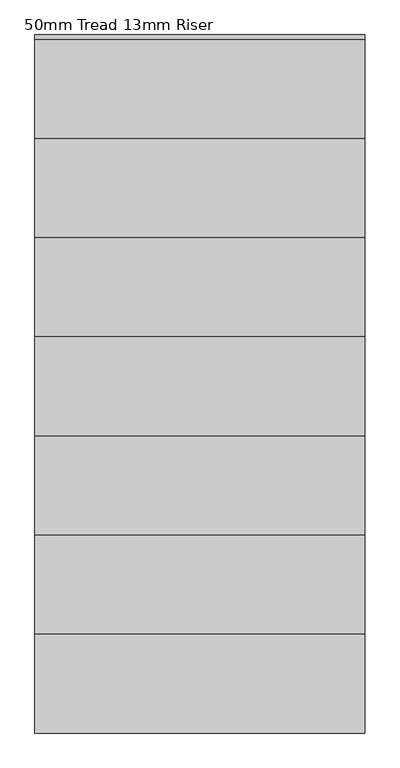
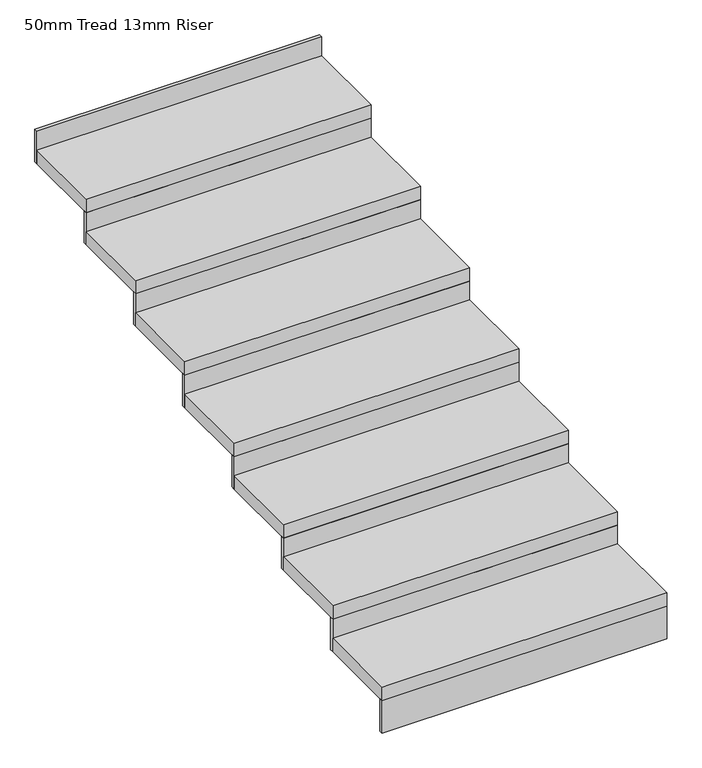
"""IFC4 building model written with IfcOpenShell, lengths in millimetres: stair flight geometry, 50mm Tread 13mm Riser."""

from ifc_helpers import new_model, si_unit, frame, origin, place, context, project, spatial, polyline, outline, extrude, source, transform, mapped, element, save


def stair_flight_50mm_tread_13mm_riser_fa5e52d7(model_context):
    return source(origin(), model_context, "Body", "SweptSolid", [
        extrude(outline(polyline([(22749.836337, -2886.2292651), (22749.836337, -2898.7292651), (21749.836337, -2898.7292651), (21749.836337, -2886.2292651), (22749.836337, -2886.2292651)])), frame((0.0, 0.0, 4630.0), z_axis=(0.0, 0.0, 1.0), x_axis=(1.0, 0.0, 0.0)), (0.0, 0.0, 1.0), 120.0),
        extrude(outline(polyline([(21749.836337, -2598.7292651), (22749.836337, -2598.7292651), (22749.836337, -2898.7292651), (21749.836337, -2898.7292651), (21749.836337, -2598.7292651)])), frame((0.0, 0.0, 4750.0), z_axis=(0.0, 0.0, 1.0), x_axis=(1.0, 0.0, 0.0)), (0.0, 0.0, 1.0), 50.0),
        extrude(outline(polyline([(22749.836337, -2586.2292651), (22749.836337, -2598.7292651), (21749.836337, -2598.7292651), (21749.836337, -2586.2292651), (22749.836337, -2586.2292651)])), frame((0.0, 0.0, 4750.0), z_axis=(0.0, 0.0, 1.0), x_axis=(1.0, 0.0, 0.0)), (0.0, 0.0, 1.0), 120.0),
        extrude(outline(polyline([(21749.836337, -2298.7292651), (22749.836337, -2298.7292651), (22749.836337, -2598.7292651), (21749.836337, -2598.7292651), (21749.836337, -2298.7292651)])), frame((0.0, 0.0, 4870.0), z_axis=(0.0, 0.0, 1.0), x_axis=(1.0, 0.0, 0.0)), (0.0, 0.0, 1.0), 50.0),
        extrude(outline(polyline([(22749.836337, -2286.2292651), (22749.836337, -2298.7292651), (21749.836337, -2298.7292651), (21749.836337, -2286.2292651), (22749.836337, -2286.2292651)])), frame((0.0, 0.0, 4870.0), z_axis=(0.0, 0.0, 1.0), x_axis=(1.0, 0.0, 0.0)), (0.0, 0.0, 1.0), 120.0),
        extrude(outline(polyline([(21749.836337, -1998.7292651), (22749.836337, -1998.7292651), (22749.836337, -2298.7292651), (21749.836337, -2298.7292651), (21749.836337, -1998.7292651)])), frame((0.0, 0.0, 4990.0), z_axis=(0.0, 0.0, 1.0), x_axis=(1.0, 0.0, 0.0)), (0.0, 0.0, 1.0), 50.0),
        extrude(outline(polyline([(22749.836337, -1986.2292651), (22749.836337, -1998.7292651), (21749.836337, -1998.7292651), (21749.836337, -1986.2292651), (22749.836337, -1986.2292651)])), frame((0.0, 0.0, 4990.0), z_axis=(0.0, 0.0, 1.0), x_axis=(1.0, 0.0, 0.0)), (0.0, 0.0, 1.0), 120.0),
        extrude(outline(polyline([(21749.836337, -1698.7292651), (22749.836337, -1698.7292651), (22749.836337, -1998.7292651), (21749.836337, -1998.7292651), (21749.836337, -1698.7292651)])), frame((0.0, 0.0, 5110.0), z_axis=(0.0, 0.0, 1.0), x_axis=(1.0, 0.0, 0.0)), (0.0, 0.0, 1.0), 50.0),
        extrude(outline(polyline([(22749.836337, -1686.2292651), (22749.836337, -1698.7292651), (21749.836337, -1698.7292651), (21749.836337, -1686.2292651), (22749.836337, -1686.2292651)])), frame((0.0, 0.0, 5110.0), z_axis=(0.0, 0.0, 1.0), x_axis=(1.0, 0.0, 0.0)), (0.0, 0.0, 1.0), 120.0),
        extrude(outline(polyline([(21749.836337, -1398.7292651), (22749.836337, -1398.7292651), (22749.836337, -1698.7292651), (21749.836337, -1698.7292651), (21749.836337, -1398.7292651)])), frame((0.0, 0.0, 5230.0), z_axis=(0.0, 0.0, 1.0), x_axis=(1.0, 0.0, 0.0)), (0.0, 0.0, 1.0), 50.0),
        extrude(outline(polyline([(22749.836337, -1386.2292651), (22749.836337, -1398.7292651), (21749.836337, -1398.7292651), (21749.836337, -1386.2292651), (22749.836337, -1386.2292651)])), frame((0.0, 0.0, 5230.0), z_axis=(0.0, 0.0, 1.0), x_axis=(1.0, 0.0, 0.0)), (0.0, 0.0, 1.0), 120.0),
        extrude(outline(polyline([(21749.836337, -1098.7292651), (22749.836337, -1098.7292651), (22749.836337, -1398.7292651), (21749.836337, -1398.7292651), (21749.836337, -1098.7292651)])), frame((0.0, 0.0, 5350.0), z_axis=(0.0, 0.0, 1.0), x_axis=(1.0, 0.0, 0.0)), (0.0, 0.0, 1.0), 50.0),
        extrude(outline(polyline([(22749.836337, -1086.2292651), (22749.836337, -1098.7292651), (21749.836337, -1098.7292651), (21749.836337, -1086.2292651), (22749.836337, -1086.2292651)])), frame((0.0, 0.0, 5350.0), z_axis=(0.0, 0.0, 1.0), x_axis=(1.0, 0.0, 0.0)), (0.0, 0.0, 1.0), 120.0),
        extrude(outline(polyline([(21749.836337, -798.7292651), (22749.836337, -798.7292651), (22749.836337, -1098.7292651), (21749.836337, -1098.7292651), (21749.836337, -798.7292651)])), frame((0.0, 0.0, 5470.0), z_axis=(0.0, 0.0, 1.0), x_axis=(1.0, 0.0, 0.0)), (0.0, 0.0, 1.0), 50.0),
        extrude(outline(polyline([(22749.836337, -786.2292651), (22749.836337, -798.7292651), (21749.836337, -798.7292651), (21749.836337, -786.2292651), (22749.836337, -786.2292651)])), frame((0.0, 0.0, 5470.0), z_axis=(0.0, 0.0, 1.0), x_axis=(1.0, 0.0, 0.0)), (0.0, 0.0, 1.0), 120.0),
    ])


if __name__ == "__main__":
    model = new_model("IFC4")
    model_context = context("Model", 3, world=origin())
    ifc_project = project(units=[si_unit("LENGTHUNIT", "METRE", prefix="MILLI")], contexts=[model_context])
    site = spatial("IfcSite", under=ifc_project)
    building = spatial("IfcBuilding", under=site)
    placement = place(None, origin())
    stair_flight_50mm_tread_13mm_riser_shape = stair_flight_50mm_tread_13mm_riser_fa5e52d7(model_context)
    element("IfcStairFlight", 1, ObjectType="50mm Tread 13mm Riser", at=placement, inside=building, context=model_context, shape_type="MappedRepresentation", body=[
        mapped(stair_flight_50mm_tread_13mm_riser_shape, transform((0.0, 0.0, 0.0), x_axis=(1.0, 0.0, 0.0), y_axis=(0.0, 1.0, 0.0), z_axis=(0.0, 0.0, 1.0))),
    ])
    save(model, "model.ifc")
